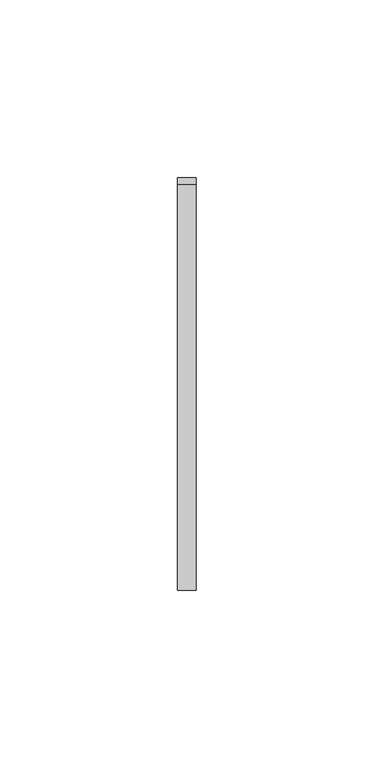
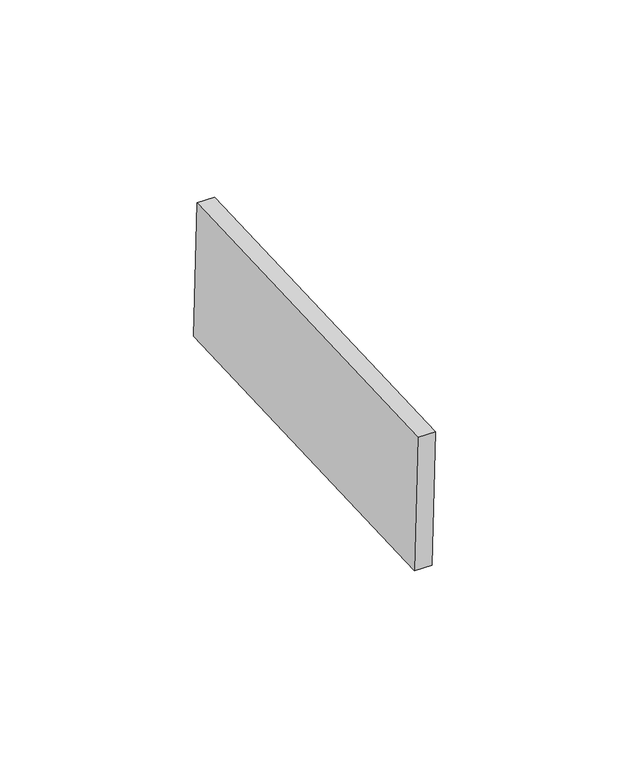
"""IFC4 building model written with IfcOpenShell, lengths in millimetres: proxy geometry, Inner panel:Inner panel:1:Inner panel:1 : Inner panel:Inner panel:300324:2:Inner panel:1:Inner panel:1 : Inner panel:Inner panel:300324:2 : Inner panel:Inner panel:1:Inner panel:1 : Inner panel:Inner panel:300324:300043:70 : Inner panel:Inner panel:1:Inner panel:1 : Inner panel:Inner panel:300324:2:Inner panel:1:Inner panel:1 : Inner panel:Inner panel:300324:2 : Inner panel:Inner panel:1:Inner panel:1 : Inner panel:Inner panel:300324:300043:308120."""

from ifc_helpers import new_model, si_unit, frame, origin, place, context, project, spatial, polyline, outline, extrude, source, transform, mapped, element, save


def generic_models_74f8cc2a(model_context):
    return source(origin(), model_context, "Body", "SweptSolid", [
        extrude(outline(polyline([(0.0, -114.2999999), (0.0, 0.0), (5.2138089, 0.0), (5.2138089, -114.2999999), (0.0, -114.2999999)])), frame((593936.595117, -576618.8219505, 4051.6214343), z_axis=(0.0, -0.04163054471216399, 0.9991330730923527), x_axis=(-1.0, 0.0, 0.0)), (0.0, 0.0, 1.0), 43.2233908),
    ])


if __name__ == "__main__":
    model = new_model("IFC4")
    model_context = context("Model", 3, world=origin())
    ifc_project = project(units=[si_unit("LENGTHUNIT", "METRE", prefix="MILLI")], contexts=[model_context])
    site = spatial("IfcSite", under=ifc_project)
    building = spatial("IfcBuilding", under=site)
    placement = place(None, origin())
    generic_models_shape = generic_models_74f8cc2a(model_context)
    element("IfcBuildingElementProxy", 1, Name="Inner panel:Inner panel:1:Inner panel:1 : Inner panel:Inner panel:300324:2:Inner panel:1:Inner panel:1 : Inner panel:Inner panel:300324:2 : Inner panel:Inner panel:1:Inner panel:1 : Inner panel:Inner panel:300324:300043:70 : Inner panel:Inner panel:1:Inner panel:1 : Inner panel:Inner panel:300324:2:Inner panel:1:Inner panel:1 : Inner panel:Inner panel:300324:2 : Inner panel:Inner panel:1:Inner panel:1 : Inner panel:Inner panel:300324:300043:308120", ObjectType="Inner panel:Inner panel:1:Inner panel:1 : Inner panel:Inner panel:300324:2:Inner panel:1:Inner panel:1 : Inner panel:Inner panel:300324:2 : Inner panel:Inner panel:1:Inner panel:1 : Inner panel:Inner panel:300324:300043:70 : Inner panel:Inner panel:1:Inner panel:1 : Inner panel:Inner panel:300324:2:Inner panel:1:Inner panel:1 : Inner panel:Inner panel:300324:2 : Inner panel:Inner panel:1:Inner panel:1 : Inner panel:Inner panel:300324:300043:308120", at=placement, inside=building, context=model_context, shape_type="MappedRepresentation", body=[
        mapped(generic_models_shape, transform((0.0, 0.0, 0.0), x_axis=(1.0, 0.0, 0.0), y_axis=(0.0, 1.0, 0.0), z_axis=(0.0, 0.0, 1.0))),
    ])
    save(model, "model.ifc")

# Revit data of these elements
# Type "Inner panel:Inner panel:1:Inner panel:1 : Inner panel:Inner panel:300324:2:Inner panel:1:Inner panel:1 : Inner panel:Inner panel:300324:2 : Inner panel:Inner panel:1:Inner panel:1 : Inner panel:Inner panel:300324:300043:70 : Inner panel:Inner panel:1:Inner panel:1 : Inner panel:Inner panel:300324:2:Inner panel:1:Inner panel:1 : Inner panel:Inner panel:300324:2 : Inner panel:Inner panel:1:Inner panel:1 : Inner panel:Inner panel:300324:300043:308120"
#   NameOverride = "Inner panel:Inner panel:1:Inner panel:1 : Inner panel:Inner panel:300324:2:Inner panel:1:Inner panel:1 : Inner panel:Inner panel:300324:2 : Inner panel:Inner panel:1:Inner panel:1 : Inner panel:Inner panel:300324:300043:308120"
#   ObjectTypeOverride = "Inner panel:1:Inner panel:1 : Inner panel:Inner panel:300324:2 : Inner panel:Inner panel:1:Inner panel:1 : Inner panel:Inner panel:300324:300043"
#   Reference = "Inner panel"
#   Tag = "308120"
# Element 1 (IfcBuildingElementProxy, "Inner panel:Inner panel:1:Inner panel:1 : Inner panel:Inner panel:300324:2:Inner panel:1:Inner panel:1 : Inner panel:Inner panel:300324:2 : Inner panel:Inner panel:1:Inner panel:1 : Inner panel:Inner panel:300324:300043:70 : Inner panel:Inner panel:1:Inner panel:1 : Inner panel:Inner panel:300324:2:Inner panel:1:Inner panel:1 : Inner panel:Inner panel:300324:2 : Inner panel:Inner panel:1:Inner panel:1 : Inner panel:Inner panel:300324:300043:308120")
#   Materials on its faces: "SLIDING CLIP"
# Materials
#   "SLIDING CLIP": class "Generic", colour RGB 120 120 120, transparency 0, Cost = 0
